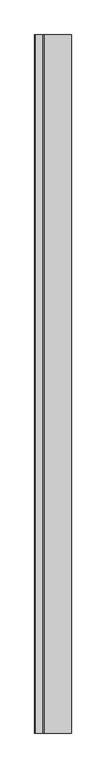
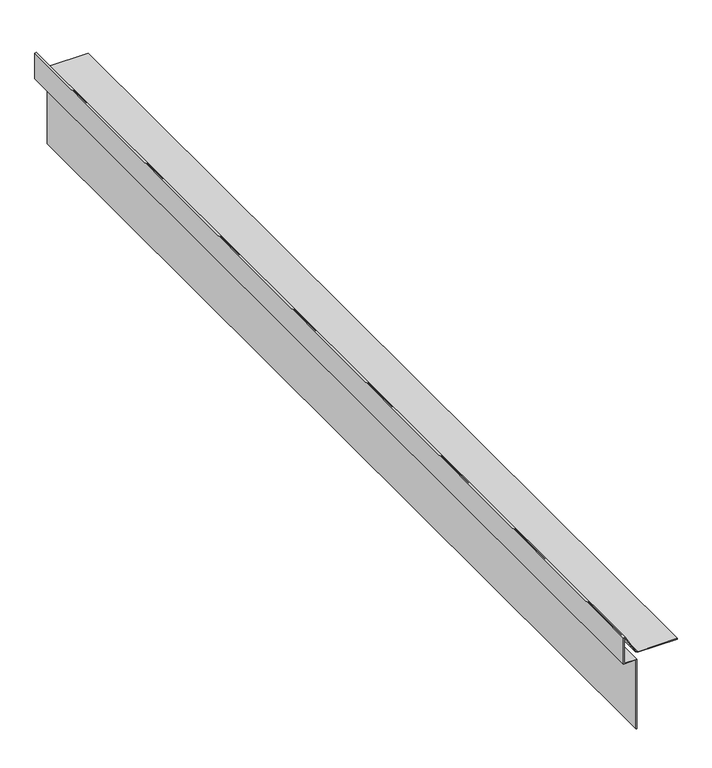
"""IFC4 building model written with IfcOpenShell, lengths in millimetres: proxy geometry, GRAVEL STOP15:GRAVEL STOP002:305334 : GRAVEL STOP15:GRAVEL STOP002:305334."""

from ifc_helpers import new_model, si_unit, frame, origin, place, context, project, spatial, polyline, outline, extrude, source, transform, mapped, element, save


def generic_models_d56acce8(model_context):
    return source(origin(), model_context, "Body", "SweptSolid", [
        extrude(outline(polyline([(40259.5408757, 1993.3009663), (40295.3431515, 1972.6305128), (40294.5307525, 1969.5985985), (40240.9633674, 1969.5985985), (40240.9633674, 1993.938336), (40097.9858473, 1993.938336), (40097.9858473, 1995.349447), (40242.3744784, 1995.349447), (40242.3744784, 1971.0097095), (40293.447969, 1971.0097095), (40293.699878, 1971.9498466), (40258.5078708, 1992.2679614), (40255.9633674, 1996.6751705), (40255.9633674, 2074.5111832), (40257.3744784, 2074.5111832), (40257.3744784, 1997.0532766), (40259.5408757, 1993.3009663)])), frame((0.0, -774.5581162, 0.0), z_axis=(0.0, 1.0, 0.0), x_axis=(0.0, 0.0, 1.0)), (0.0, 0.0, 1.0), 2000.25),
    ])


if __name__ == "__main__":
    model = new_model("IFC4")
    model_context = context("Model", 3, world=origin())
    ifc_project = project(units=[si_unit("LENGTHUNIT", "METRE", prefix="MILLI")], contexts=[model_context])
    site = spatial("IfcSite", under=ifc_project)
    building = spatial("IfcBuilding", under=site)
    placement = place(None, origin())
    generic_models_shape = generic_models_d56acce8(model_context)
    element("IfcBuildingElementProxy", 1, Name="GRAVEL STOP15:GRAVEL STOP002:305334 : GRAVEL STOP15:GRAVEL STOP002:305334", ObjectType="GRAVEL STOP15:GRAVEL STOP002:305334 : GRAVEL STOP15:GRAVEL STOP002:305334", at=placement, inside=building, context=model_context, shape_type="MappedRepresentation", body=[
        mapped(generic_models_shape, transform((0.0, 0.0, 0.0), x_axis=(1.0, 0.0, 0.0), y_axis=(0.0, 1.0, 0.0), z_axis=(0.0, 0.0, 1.0))),
    ])
    save(model, "model.ifc")

# Revit data of these elements
# Type "GRAVEL STOP15:GRAVEL STOP002:305334 : GRAVEL STOP15:GRAVEL STOP002:305334"
#   NameOverride = "GRAVEL STOP15:GRAVEL STOP002:305334"
#   ObjectTypeOverride = "GRAVEL STOP15:GRAVEL STOP002"
#   Reference = "GRAVEL STOP002"
#   Category = "Generic Models"
#   Tag = "305334"
# Element 1 (IfcBuildingElementProxy, "GRAVEL STOP15:GRAVEL STOP002:305334 : GRAVEL STOP15:GRAVEL STOP002:305334")
#   Materials on its faces: "GRAVEL STOP REQUIRED WITH GRAVEL SURFACE SYSTEMS"
# Materials
#   "GRAVEL STOP REQUIRED WITH GRAVEL SURFACE SYSTEMS": class "Unassigned", colour RGB 170 170 127, transparency 0, Cost = 0
